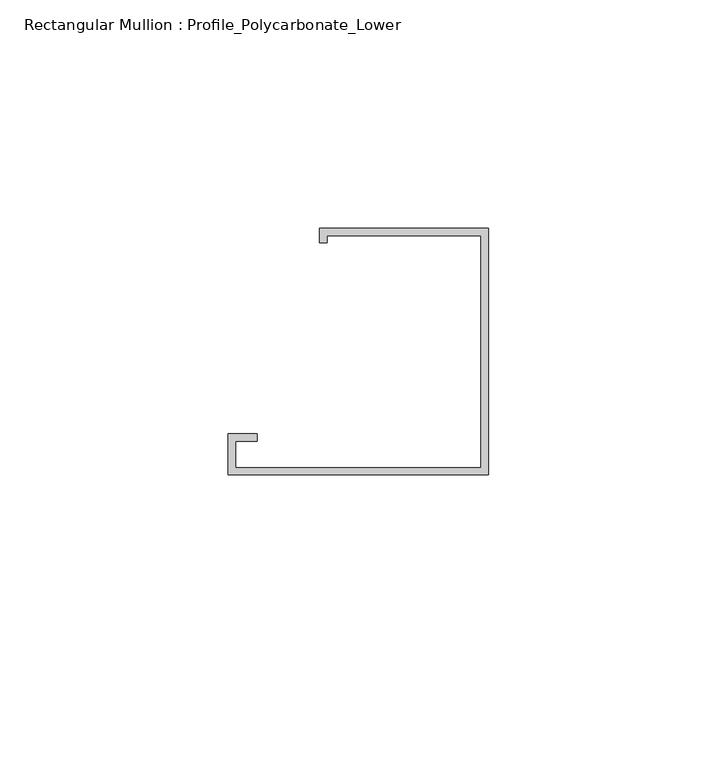
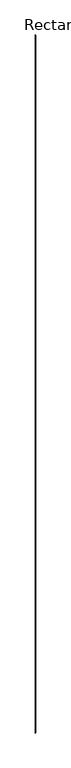
"""IFC4 building model written with IfcOpenShell, lengths in millimetres: member geometry, Rectangular Mullion : Profile_Polycarbonate_Lower."""

from ifc_helpers import new_model, si_unit, frame, origin, place, context, project, spatial, polyline, outline, extrude, source, transform, mapped, element, save


def rectangular_mullion_profile_polycarbonate_lower_125f09d9(model_context):
    return source(origin(), model_context, "Body", "SweptSolid", [
        extrude(outline(polyline([(0.0, -28.984575), (-56.9976, -28.984575), (-56.9976, -19.992975), (-50.6476, -19.992975), (-50.6476, -21.580475), (-55.4101, -21.580475), (-55.4101, -27.397075), (-1.5875, -27.397075), (-1.5875, 23.428325), (-35.3949, 23.428325), (-35.3949, 21.840825), (-36.9824, 21.840825), (-36.9824, 25.015825), (0.0, 25.015825), (0.0, -28.984575)])), frame((0.0, 0.0, -81115.1885281), z_axis=(0.0, 0.0, 1.0), x_axis=(1.0, 0.0, 0.0)), (0.0, 0.0, 1.0), 81115.1885281),
    ])


if __name__ == "__main__":
    model = new_model("IFC4")
    model_context = context("Model", 3, world=origin())
    ifc_project = project(units=[si_unit("LENGTHUNIT", "METRE", prefix="MILLI")], contexts=[model_context])
    site = spatial("IfcSite", under=ifc_project)
    building = spatial("IfcBuilding", under=site)
    placement = place(None, origin())
    rectangular_mullion_profile_polycarbonate_lower_shape = rectangular_mullion_profile_polycarbonate_lower_125f09d9(model_context)
    element("IfcMember", 1, ObjectType="Rectangular Mullion : Profile_Polycarbonate_Lower", at=placement, inside=building, context=model_context, shape_type="MappedRepresentation", body=[
        mapped(rectangular_mullion_profile_polycarbonate_lower_shape, transform((0.0, 0.0, 0.0), x_axis=(1.0, 0.0, 0.0), y_axis=(0.0, 1.0, 0.0), z_axis=(0.0, 0.0, 1.0))),
    ])
    save(model, "model.ifc")

# Revit data of these elements
# Type "Rectangular Mullion : Profile_Polycarbonate_Lower"
#   built-in parameter 1007322 = 0.177167 (stored number, unit not read)
#   built-in parameter 1007321 = 0 (stored number, unit not read)
#   built-in parameter 1007320 = 0.00520833 (stored number, unit not read)
